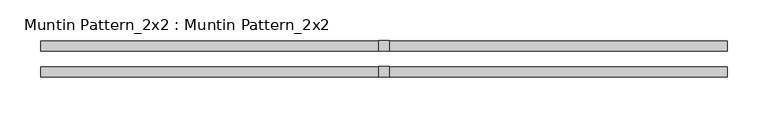
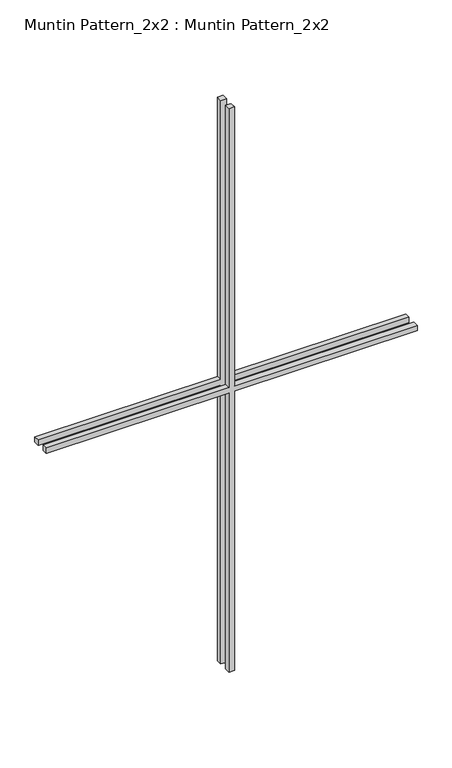
"""IFC4 building model written with IfcOpenShell, lengths in millimetres: proxy geometry, Muntin Pattern_2x2 : Muntin Pattern_2x2."""

import ifcopenshell
import ifcopenshell.guid

model = None  # the IFC model being written
_history = None  # IfcOwnerHistory: only IFC2X3 demands one
_inside = {}  # id of a spatial element -> (the spatial element, [elements in it])
_under = {}  # id of a project, library or spatial element -> (it, [spatial elements below it])
_declared = {}  # id of a project -> (the project, [libraries it declares])
_typed = {}  # id of a type object -> (the type object, [elements of that type])
_made_of = {}  # id of a material, layer set ... -> (it, [elements and type objects made of it])


def new_model(schema):
    """Start an empty IFC model of exactly this schema.

    Asked for "IFC4X3", IfcOpenShell would pick the latest addendum, in which some entities
    have other attributes; the version numbers below select the first issue.
    IFC2X3 requires an IfcOwnerHistory on every rooted entity: one is made here for all.
    """
    global model, _history
    if schema == "IFC4X3":
        model = ifcopenshell.file(schema_version=(4, 3, 0, 0))
    else:
        model = ifcopenshell.file(schema=schema)
    _inside.clear()
    _under.clear()
    _declared.clear()
    _typed.clear()
    _made_of.clear()
    _history = None
    if model.schema == "IFC2X3":
        org = make("IfcOrganization", Name="unknown")
        user = make(
            "IfcPersonAndOrganization",
            ThePerson=make("IfcPerson", FamilyName="unknown"),
            TheOrganization=org,
        )
        app = make(
            "IfcApplication",
            ApplicationDeveloper=org,
            Version="unknown",
            ApplicationFullName="unknown",
            ApplicationIdentifier="unknown",
        )
        _history = make(
            "IfcOwnerHistory",
            OwningUser=user,
            OwningApplication=app,
            ChangeAction="ADDED",
            CreationDate=0,
        )
    return model


def make(cls, **values):
    """One entity of the class cls with the attributes given. An attribute that is None is left unset."""
    return model.create_entity(
        cls, **{name: value for name, value in values.items() if value is not None}
    )


def rooted(cls, **values):
    """An entity with a GlobalId (a new one), such as an element, a storey or a relation."""
    return make(cls, GlobalId=ifcopenshell.guid.new(), OwnerHistory=_history, **values)


def si_unit(unit_type, name, prefix=None):
    """IfcSIUnit, for example si_unit("LENGTHUNIT", "METRE", prefix="MILLI")."""
    return make("IfcSIUnit", UnitType=unit_type, Prefix=prefix, Name=name)


def assignment(units):
    """IfcUnitAssignment: the units of a project."""
    return None if units is None else make("IfcUnitAssignment", Units=units)


def point(xyz):
    """IfcCartesianPoint."""
    return None if xyz is None else make("IfcCartesianPoint", Coordinates=xyz)


def direction(xyz):
    """IfcDirection."""
    return None if xyz is None else make("IfcDirection", DirectionRatios=xyz)


def frame(location, z_axis=None, x_axis=None):
    """IfcAxis2Placement3D, a coordinate frame: its origin and axes. An axis left out is left unset."""
    return make(
        "IfcAxis2Placement3D",
        Location=point(location),
        Axis=direction(z_axis),
        RefDirection=direction(x_axis),
    )


def origin():
    """The frame at (0, 0, 0) with its axes left unset."""
    return frame((0.0, 0.0, 0.0))


def place(relative_to, where):
    """IfcLocalPlacement: puts the frame where relative to a parent placement (None: the world)."""
    return make(
        "IfcLocalPlacement", PlacementRelTo=relative_to, RelativePlacement=where
    )


def context(
    kind, dimensions, precision=None, world=None, true_north=None, identifier=None
):
    """IfcGeometricRepresentationContext, for example the 3D "Model" context."""
    return make(
        "IfcGeometricRepresentationContext",
        ContextIdentifier=identifier,
        ContextType=kind,
        CoordinateSpaceDimension=dimensions,
        Precision=precision,
        WorldCoordinateSystem=world,
        TrueNorth=true_north,
    )


def project(units=None, contexts=None):
    """IfcProject with its units and contexts."""
    return rooted(
        "IfcProject",
        Name="project",
        RepresentationContexts=contexts,
        UnitsInContext=assignment(units),
    )


def spatial(cls, under=None, at=None, **own):
    """A site, building, storey or space (cls), placed at a placement, below another one or the project."""
    s = rooted(cls, ObjectPlacement=at, **own)
    if under is not None:
        _under.setdefault(under.id(), (under, []))[1].append(s)
    return s


def polyline(points):
    """IfcPolyline through the points."""
    return make("IfcPolyline", Points=[point(p) for p in points])


def outline(outer, holes=None, kind="AREA"):
    """IfcArbitraryClosedProfileDef: a profile drawn as a closed curve; with holes, ...WithVoids."""
    if holes is None:
        return make("IfcArbitraryClosedProfileDef", ProfileType=kind, OuterCurve=outer)
    return make(
        "IfcArbitraryProfileDefWithVoids",
        ProfileType=kind,
        OuterCurve=outer,
        InnerCurves=holes,
    )


def extrude(swept, where, along, depth):
    """IfcExtrudedAreaSolid: the profile swept, set in the frame where, extruded along a direction by depth."""
    return make(
        "IfcExtrudedAreaSolid",
        SweptArea=swept,
        Position=where,
        ExtrudedDirection=direction(along),
        Depth=depth,
    )


def shape(context_of_items, identifier, shape_type, items):
    """IfcShapeRepresentation: the items that make up one representation, for example the "Body"."""
    return make(
        "IfcShapeRepresentation",
        ContextOfItems=context_of_items,
        RepresentationIdentifier=identifier,
        RepresentationType=shape_type,
        Items=items,
    )


def source(mapping_origin, context_of_items, identifier, shape_type, items):
    """IfcRepresentationMap: a shape defined once, which mapped items show again and again."""
    return make(
        "IfcRepresentationMap",
        MappingOrigin=mapping_origin,
        MappedRepresentation=shape(context_of_items, identifier, shape_type, items),
    )


def transform(
    local_origin,
    x_axis=None,
    y_axis=None,
    z_axis=None,
    scale=None,
    scale2=None,
    scale3=None,
    uniform=True,
):
    """IfcCartesianTransformationOperator3D, or its non-uniform kind. x_axis, y_axis, z_axis: its Axis1, 2, 3."""
    if uniform:
        return make(
            "IfcCartesianTransformationOperator3D",
            Axis1=direction(x_axis),
            Axis2=direction(y_axis),
            LocalOrigin=point(local_origin),
            Scale=scale,
            Axis3=direction(z_axis),
        )
    return make(
        "IfcCartesianTransformationOperator3DnonUniform",
        Axis1=direction(x_axis),
        Axis2=direction(y_axis),
        LocalOrigin=point(local_origin),
        Scale=scale,
        Axis3=direction(z_axis),
        Scale2=scale2,
        Scale3=scale3,
    )


def mapped(mapping_source, mapping_target):
    """IfcMappedItem: shows the shape of a source again, moved by a transform."""
    return make(
        "IfcMappedItem", MappingSource=mapping_source, MappingTarget=mapping_target
    )


def made_of(thing, what):
    """Note that an element or type object is made of a material, layer set ...; save() writes the relation."""
    if what is not None:
        _made_of.setdefault(what.id(), (what, []))[1].append(thing)
    return thing


def element(
    cls,
    number,
    at=None,
    inside=None,
    cuts=None,
    type_object=None,
    material=None,
    context=None,
    identifier="Body",
    shape_type=None,
    held_by="IfcProductDefinitionShape",
    body=None,
    shapes=None,
    **own,
):
    """One element of the class cls, such as IfcWall. Its Tag is "e" and its number.

    at: its placement. inside: the storey or other place that contains it. cuts: it is an
    opening in that element (IfcRelVoidsElement). A single representation is given by context,
    identifier, shape_type and body (its items); several are given by shapes. held_by: the class
    of the entity that holds the representations. save() writes the other relations.
    """
    e = rooted(cls, Tag="e%d" % number, ObjectPlacement=at, **own)
    if body is not None:
        shapes = [shape(context, identifier, shape_type, body)]
    if shapes is not None:
        e.Representation = make(held_by, Representations=shapes)
    if inside is not None:
        _inside.setdefault(inside.id(), (inside, []))[1].append(e)
    if cuts is not None:
        rooted(
            "IfcRelVoidsElement", RelatingBuildingElement=cuts, RelatedOpeningElement=e
        )
    if type_object is not None:
        _typed.setdefault(type_object.id(), (type_object, []))[1].append(e)
    return made_of(e, material)


def aggregate(whole, parts):
    """IfcRelAggregates: a whole, such as a stair, and the parts it consists of."""
    return rooted("IfcRelAggregates", RelatingObject=whole, RelatedObjects=parts)


def save(model, path):
    """Write the relations noted so far, then the file.

    IfcRelAggregates (storeys below a building ...), IfcRelContainedInSpatialStructure (elements
    in a storey), IfcRelDefinesByType, IfcRelAssociatesMaterial and IfcRelDeclares: one each for
    every whole, place, type object, material and project.
    """
    for whole, parts in _under.values():
        aggregate(whole, parts)
    for where, things in _inside.values():
        rooted(
            "IfcRelContainedInSpatialStructure",
            RelatedElements=things,
            RelatingStructure=where,
        )
    for kind, things in _typed.values():
        rooted("IfcRelDefinesByType", RelatedObjects=things, RelatingType=kind)
    for what, things in _made_of.values():
        rooted("IfcRelAssociatesMaterial", RelatedObjects=things, RelatingMaterial=what)
    for by, libraries in _declared.values():
        rooted("IfcRelDeclares", RelatingContext=by, RelatedDefinitions=libraries)
    model.write(path)


def muntin_pattern_2x2_muntin_pattern_2x2_66e60b0d(model_context):
    return source(origin(), model_context, "Body", "SweptSolid", [
        extrude(outline(polyline([(679.45, -6.35), (679.45, -419.1), (666.75, -419.1), (666.75, -6.35), (0.0, -6.35), (0.0, 6.35), (666.75, 6.35), (666.75, 419.1), (679.45, 419.1), (679.45, 6.35), (1346.2, 6.35), (1346.2, -6.35), (679.45, -6.35)])), frame((0.0, 9.525, 0.0), z_axis=(0.0, 1.0, 0.0), x_axis=(0.0, 0.0, 1.0)), (0.0, 0.0, 1.0), 12.7),
        extrude(outline(polyline([(679.45, -6.35), (679.45, -419.1), (666.75, -419.1), (666.75, -6.35), (0.0, -6.35), (0.0, 6.35), (666.75, 6.35), (666.75, 419.1), (679.45, 419.1), (679.45, 6.35), (1346.2, 6.35), (1346.2, -6.35), (679.45, -6.35)])), frame((0.0, -22.225, 0.0), z_axis=(0.0, 1.0, 0.0), x_axis=(0.0, 0.0, 1.0)), (0.0, 0.0, 1.0), 12.7),
    ])


if __name__ == "__main__":
    model = new_model("IFC4")
    model_context = context("Model", 3, world=origin())
    ifc_project = project(units=[si_unit("LENGTHUNIT", "METRE", prefix="MILLI")], contexts=[model_context])
    site = spatial("IfcSite", under=ifc_project)
    building = spatial("IfcBuilding", under=site)
    placement = place(None, origin())
    muntin_pattern_2x2_muntin_pattern_2x2_shape = muntin_pattern_2x2_muntin_pattern_2x2_66e60b0d(model_context)
    element("IfcBuildingElementProxy", 1, Name="Muntin Pattern_2x2 : Muntin Pattern_2x2", ObjectType="Muntin Pattern_2x2 : Muntin Pattern_2x2", at=placement, inside=building, context=model_context, shape_type="MappedRepresentation", body=[
        mapped(muntin_pattern_2x2_muntin_pattern_2x2_shape, transform((0.0, 0.0, 0.0), x_axis=(1.0, 0.0, 0.0), y_axis=(0.0, 1.0, 0.0), z_axis=(0.0, 0.0, 1.0))),
    ])
    save(model, "model.ifc")

# Revit data of these elements
# Type "Muntin Pattern_2x2 : Muntin Pattern_2x2"
#   Width [instance default] = 4' - 0"
#   Thickness = 0' - 0 1/2"
#   Height [instance default] = 4' - 0"
#   Distance = 0' - 0 3/4"
#   Interior Material [instance default] = none
#   Exterior Material [instance default] = none
#   Default Elevation = 0
# Element 1 (IfcBuildingElementProxy, "Muntin Pattern_2x2 : Muntin Pattern_2x2")
#   Width = 2' - 9"
#   Height = 4' - 5"
#   Interior Material = Wood - Stained
#   Exterior Material = Clad - White
#   Materials on its faces: "Clad - White", "Wood - Stained"
# Materials
#   "Clad - White": class "Wood", colour RGB 242 242 238, transparency 0, Cost = 0
#   "Wood - Stained": class "Wood", colour RGB 224 178 126, transparency 0, Cost = 0
